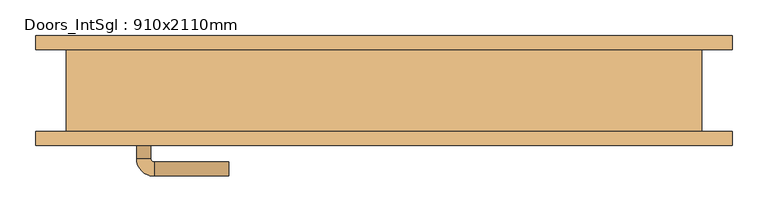
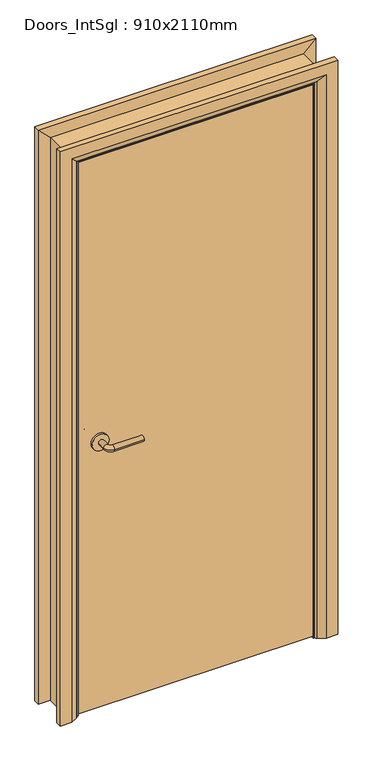
"""IFC4 building model written with IfcOpenShell, lengths in millimetres: door geometry, Doors_IntSgl : 910x2110mm."""

from ifc_helpers import new_model, si_unit, point, frame, frame_2d, origin, place, context, project, spatial, polyline, circle_curve, ellipse_curve, trimmed, segment, composite_curve, outline, extrude, faceted_brep, source, transform, mapped, element, save
from ifc_brep_helpers import plane_surface, cylinder_surface, revolved_surface, advanced_brep


def doors_intsgl_910x2110mm_d0108889(model_context):
    return source(origin(), model_context, "Body", "SolidModel", [
        advanced_brep(
        [(-348.0, -11.5, 1000.0), (-328.0, -11.5, 1000.0), (-348.0, 18.5, 1000.0), (-328.0, 18.5, 1000.0), (-323.0, 23.5, 1000.0), (-323.0, 43.5, 1000.0), (-218.0, 43.5, 1000.0), (-218.0, 23.5, 1000.0)],
        [
            (0, 1, circle_curve(frame((-338.0, -11.5, 1000.0), z_axis=(0.0, -1.0, 0.0), x_axis=(1.0, 0.0, 0.0)), 10.0)),
            (1, 0, circle_curve(frame((-338.0, -11.5, 1000.0), z_axis=(0.0, -1.0, 0.0), x_axis=(1.0, 0.0, 0.0)), 10.0)),
            (0, 2),
            (2, 3, circle_curve(frame((-338.0, 18.5, 1000.0), z_axis=(0.0, -1.0, 0.0), x_axis=(1.0, 0.0, 0.0)), 10.0)),
            (3, 1),
            (3, 2, circle_curve(frame((-338.0, 18.5, 1000.0), z_axis=(0.0, -1.0, 0.0), x_axis=(1.0, 0.0, 0.0)), 10.0)),
            (4, 3, circle_curve(frame((-323.0, 18.5, 1000.0), z_axis=(0.0, 0.0, 1.0), x_axis=(-1.0, 0.0, 0.0)), 5.0)),
            (2, 5, circle_curve(frame((-323.0, 18.5, 1000.0), z_axis=(0.0, 0.0, -1.0), x_axis=(-1.0, 0.0, 0.0)), 25.0)),
            (5, 4, circle_curve(frame((-323.0, 33.5, 1000.0), z_axis=(-1.0, 0.0, 0.0), x_axis=(0.0, -1.0, 0.0)), 10.0)),
            (4, 5, circle_curve(frame((-323.0, 33.5, 1000.0), z_axis=(-1.0, 0.0, 0.0), x_axis=(0.0, -1.0, 0.0)), 10.0)),
            (6, 7, circle_curve(frame((-218.0, 33.5, 1000.0), z_axis=(1.0, 0.0, 0.0), x_axis=(0.0, -1.0, 0.0)), 10.0)),
            (7, 6, circle_curve(frame((-218.0, 33.5, 1000.0), z_axis=(1.0, 0.0, 0.0), x_axis=(0.0, -1.0, 0.0)), 10.0)),
            (5, 6),
            (7, 4),
        ],
        [
            plane_surface(frame((-338.0, -11.5, 1000.0), z_axis=(0.0, -1.0, 0.0), x_axis=(0.0, 0.0, 1.0))),
            cylinder_surface(frame((-338.0, -11.5, 1000.0), z_axis=(0.0, -1.0, 0.0), x_axis=(1.0, 0.0, 0.0)), 10.0),
            revolved_surface(trimmed(ellipse_curve(frame((-338.0, 18.5, 1000.0), z_axis=(0.0, -1.0, 0.0), x_axis=(1.0, 0.0, 0.0)), 10.0, 10.0), [point((-348.0, 18.5, 1000.0))], [point((-328.0, 18.5, 1000.0))], True, "CARTESIAN"), (-323.0, 18.5, 1000.0), (0.0, 0.0, -1.0)),
            revolved_surface(trimmed(ellipse_curve(frame((-338.0, 18.5, 1000.0), z_axis=(0.0, -1.0, 0.0), x_axis=(1.0, 0.0, 0.0)), 10.0, 10.0), [point((-328.0, 18.5, 1000.0))], [point((-348.0, 18.5, 1000.0))], True, "CARTESIAN"), (-323.0, 18.5, 1000.0), (0.0, 0.0, -1.0)),
            plane_surface(frame((-218.0, 33.5, 1000.0), z_axis=(1.0, 0.0, 0.0), x_axis=(0.0, 0.0, 1.0))),
            cylinder_surface(frame((-323.0, 33.5, 1000.0), z_axis=(-1.0, 0.0, 0.0), x_axis=(0.0, -1.0, 0.0)), 10.0),
        ],
        [
            (0, [[1, 2]]),
            (1, [[-1, 3, 4, 5]]),
            (1, [[-2, -5, 6, -3]]),
            (2, [[7, -4, 8, 9]]),
            (3, [[-8, -6, -7, 10]]),
            (4, [[11, 12]]),
            (5, [[-9, 13, -12, 14]]),
            (5, [[-10, -14, -11, -13]]),
        ],
    ),
        extrude(outline(composite_curve([segment(trimmed(circle_curve(frame_2d((1000.0, -340.5)), 30.0), [point((1000.0, -370.5))], [point((1000.0, -310.5))], False, "CARTESIAN"), True, "CONTINUOUS"), segment(trimmed(circle_curve(frame_2d((1000.0, -340.5)), 30.0), [point((1000.0, -310.5))], [point((1000.0, -370.5))], False, "CARTESIAN"), True, "CONTINUOUS")], self_intersect=False)), frame((0.0, -19.5, 0.0), z_axis=(0.0, 1.0, 0.0), x_axis=(0.0, 0.0, 1.0)), (0.0, 0.0, 1.0), 8.0),
        advanced_brep(
        [(-348.0, -65.5, 1000.0), (-328.0, -65.5, 1000.0), (-328.0, -95.5, 1000.0), (-348.0, -95.5, 1000.0), (-323.0, -100.5, 1000.0), (-323.0, -120.5, 1000.0), (-218.0, -120.5, 1000.0), (-218.0, -100.5, 1000.0)],
        [
            (0, 1, circle_curve(frame((-338.0, -65.5, 1000.0), z_axis=(0.0, 1.0, 0.0), x_axis=(1.0, 0.0, 0.0)), 10.0)),
            (1, 0, circle_curve(frame((-338.0, -65.5, 1000.0), z_axis=(0.0, 1.0, 0.0), x_axis=(1.0, 0.0, 0.0)), 10.0)),
            (1, 2),
            (2, 3, circle_curve(frame((-338.0, -95.5, 1000.0), z_axis=(0.0, 1.0, 0.0), x_axis=(1.0, 0.0, 0.0)), 10.0)),
            (3, 0),
            (3, 2, circle_curve(frame((-338.0, -95.5, 1000.0), z_axis=(0.0, 1.0, 0.0), x_axis=(1.0, 0.0, 0.0)), 10.0)),
            (4, 5, circle_curve(frame((-323.0, -110.5, 1000.0), z_axis=(-1.0, 0.0, 0.0), x_axis=(0.0, 1.0, 0.0)), 10.0)),
            (5, 3, circle_curve(frame((-323.0, -95.5, 1000.0), z_axis=(0.0, 0.0, -1.0), x_axis=(-1.0, 0.0, 0.0)), 25.0)),
            (2, 4, circle_curve(frame((-323.0, -95.5, 1000.0), z_axis=(0.0, 0.0, 1.0), x_axis=(-1.0, 0.0, 0.0)), 5.0)),
            (5, 4, circle_curve(frame((-323.0, -110.5, 1000.0), z_axis=(-1.0, 0.0, 0.0), x_axis=(0.0, 1.0, 0.0)), 10.0)),
            (6, 7, circle_curve(frame((-218.0, -110.5, 1000.0), z_axis=(1.0, 0.0, 0.0), x_axis=(0.0, 1.0, 0.0)), 10.0)),
            (7, 6, circle_curve(frame((-218.0, -110.5, 1000.0), z_axis=(1.0, 0.0, 0.0), x_axis=(0.0, 1.0, 0.0)), 10.0)),
            (4, 7),
            (6, 5),
        ],
        [
            plane_surface(frame((-338.0, -65.5, 1000.0), z_axis=(0.0, 1.0, 0.0), x_axis=(0.0, 0.0, 1.0))),
            cylinder_surface(frame((-338.0, -65.5, 1000.0), z_axis=(0.0, 1.0, 0.0), x_axis=(1.0, 0.0, 0.0)), 10.0),
            revolved_surface(trimmed(ellipse_curve(frame((-338.0, -95.5, 1000.0), z_axis=(0.0, -1.0, 0.0), x_axis=(1.0, 0.0, 0.0)), 10.0, 10.0), [point((-348.0, -95.5, 1000.0))], [point((-328.0, -95.5, 1000.0))], True, "CARTESIAN"), (-323.0, -95.5, 1000.0), (0.0, 0.0, -1.0)),
            revolved_surface(trimmed(ellipse_curve(frame((-338.0, -95.5, 1000.0), z_axis=(0.0, -1.0, 0.0), x_axis=(1.0, 0.0, 0.0)), 10.0, 10.0), [point((-328.0, -95.5, 1000.0))], [point((-348.0, -95.5, 1000.0))], True, "CARTESIAN"), (-323.0, -95.5, 1000.0), (0.0, 0.0, -1.0)),
            plane_surface(frame((-218.0, -110.5, 1000.0), z_axis=(1.0, 0.0, 0.0), x_axis=(0.0, 0.0, 1.0))),
            cylinder_surface(frame((-323.0, -110.5, 1000.0), z_axis=(-1.0, 0.0, 0.0), x_axis=(0.0, 1.0, 0.0)), 10.0),
        ],
        [
            (0, [[1, 2]]),
            (1, [[3, 4, 5, -2]]),
            (1, [[-5, 6, -3, -1]]),
            (2, [[7, 8, -4, 9]]),
            (3, [[10, -9, -6, -8]]),
            (4, [[11, 12]]),
            (5, [[13, -11, 14, -7]]),
            (5, [[-14, -12, -13, -10]]),
        ],
    ),
        extrude(outline(composite_curve([segment(trimmed(circle_curve(frame_2d((1000.0, -340.5)), 30.0), [point((1000.0, -370.5))], [point((1000.0, -310.5))], False, "CARTESIAN"), True, "CONTINUOUS"), segment(trimmed(circle_curve(frame_2d((1000.0, -340.5)), 30.0), [point((1000.0, -310.5))], [point((1000.0, -370.5))], False, "CARTESIAN"), True, "CONTINUOUS")], self_intersect=False)), frame((0.0, -65.5, 0.0), z_axis=(0.0, 1.0, 0.0), x_axis=(0.0, 0.0, 1.0)), (0.0, 0.0, 1.0), 8.0),
        extrude(outline(polyline([(413.0, -19.5), (413.0, -57.5), (-413.0, -57.5), (-413.0, -19.5), (413.0, -19.5)])), frame((0.0, 0.0, 8.0), z_axis=(0.0, 0.0, 1.0), x_axis=(1.0, 0.0, 0.0)), (0.0, 0.0, 1.0), 2060.0),
        advanced_brep(
        [(490.0, -77.5, 0.0), (450.0, -77.5, 0.0), (424.0, -63.5, 0.0), (420.0, -57.5, 0.0), (490.0, -57.5, 0.0), (490.0, -57.5, 2145.0), (490.0, -77.5, 2145.0), (420.0, -57.5, 2075.0), (-420.0, -57.5, 2075.0), (-420.0, -57.5, 0.0), (-490.0, -57.5, 0.0), (-490.0, -57.5, 2145.0), (424.0, -63.5, 2079.0), (450.0, -77.5, 2105.0), (-490.0, -77.5, 2145.0), (-490.0, -77.5, 0.0), (-450.0, -77.5, 0.0), (-450.0, -77.5, 2105.0), (-424.0, -63.5, 2079.0), (-424.0, -63.5, 0.0)],
        [
            (0, 1),
            (1, 2),
            (2, 3, circle_curve(frame((428.0, -56.5, 0.0), z_axis=(0.0, 0.0, -1.0), x_axis=(1.0, 0.0, 0.0)), 8.0622577)),
            (3, 4),
            (4, 0),
            (4, 5),
            (5, 6),
            (6, 0),
            (3, 7),
            (7, 8),
            (8, 9),
            (9, 10),
            (10, 11),
            (11, 5),
            (2, 12),
            (12, 7, ellipse_curve(frame((428.0, -56.5, 2083.0), z_axis=(0.7071067811865475, 0.0, -0.7071067811865475), x_axis=(-0.7071067811865474, 0.0, -0.7071067811865476)), 11.4017543, 8.0622577)),
            (1, 13),
            (13, 12),
            (6, 14),
            (14, 15),
            (15, 16),
            (16, 17),
            (17, 13),
            (11, 14),
            (12, 18),
            (18, 8, ellipse_curve(frame((-428.0, -56.5, 2083.0), z_axis=(0.7071067811865475, 0.0, 0.7071067811865475), x_axis=(0.7071067811865476, 0.0, -0.7071067811865474)), 11.4017543, 8.0622577)),
            (17, 18),
            (15, 10),
            (9, 19, circle_curve(frame((-428.0, -56.5, 0.0), z_axis=(0.0, 0.0, -1.0), x_axis=(-1.0, 0.0, 0.0)), 8.0622577)),
            (19, 16),
            (18, 19),
        ],
        [
            plane_surface(frame((420.0, -57.5, 0.0), z_axis=(0.0, 0.0, -1.0), x_axis=(0.0, 1.0, 0.0))),
            plane_surface(frame((490.0, -77.5, 0.0), z_axis=(1.0, 0.0, 0.0), x_axis=(0.0, 0.0, 1.0))),
            plane_surface(frame((490.0, -57.5, 0.0), z_axis=(0.0, 1.0, 0.0), x_axis=(0.0, 0.0, 1.0))),
            cylinder_surface(frame((428.0, -56.5, 0.0), z_axis=(0.0, 0.0, -1.0), x_axis=(1.0, 0.0, 0.0)), 8.0622577),
            plane_surface(frame((424.0, -63.5, 0.0), z_axis=(-0.4740998230350126, -0.880471099922178, 0.0), x_axis=(0.0, 0.0, 1.0))),
            plane_surface(frame((450.0, -77.5, 0.0), z_axis=(0.0, -1.0, 0.0), x_axis=(0.0, 0.0, 1.0))),
            plane_surface(frame((490.0, -77.5, 2145.0), z_axis=(0.0, 0.0, 1.0), x_axis=(-1.0, 0.0, 0.0))),
            cylinder_surface(frame((420.0, -56.5, 2083.0), z_axis=(1.0, 0.0, 0.0), x_axis=(0.0, 0.0, 1.0)), 8.0622577),
            plane_surface(frame((424.0, -63.5, 2079.0), z_axis=(0.0, -0.8804710999221764, -0.4740998230350154), x_axis=(-1.0, 0.0, 0.0))),
            plane_surface(frame((-420.0, -57.5, 0.0), z_axis=(0.0, 0.0, -1.0), x_axis=(0.0, 1.0, 0.0))),
            plane_surface(frame((-490.0, -77.5, 2145.0), z_axis=(-1.0, 0.0, 0.0), x_axis=(0.0, 0.0, -1.0))),
            cylinder_surface(frame((-428.0, -56.5, 2075.0), z_axis=(0.0, 0.0, 1.0), x_axis=(-1.0, 0.0, 0.0)), 8.0622577),
            plane_surface(frame((-424.0, -63.5, 2079.0), z_axis=(0.47409982303501824, -0.8804710999221749, 0.0), x_axis=(0.0, 0.0, -1.0))),
        ],
        [
            (0, [[1, 2, 3, 4, 5]]),
            (1, [[6, 7, 8, -5]]),
            (2, [[9, 10, 11, 12, 13, 14, -6, -4]]),
            (3, [[15, 16, -9, -3]]),
            (4, [[17, 18, -15, -2]]),
            (5, [[-8, 19, 20, 21, 22, 23, -17, -1]]),
            (6, [[-14, 24, -19, -7]]),
            (7, [[25, 26, -10, -16]]),
            (8, [[-23, 27, -25, -18]]),
            (9, [[28, -12, 29, 30, -21]]),
            (10, [[-13, -28, -20, -24]]),
            (11, [[31, -29, -11, -26]]),
            (12, [[-22, -30, -31, -27]]),
        ],
    ),
        extrude(outline(polyline([(0.0, -396.0), (2051.0, -396.0), (2051.0, 396.0), (0.0, 396.0), (0.0, 415.0), (2070.0, 415.0), (2070.0, -415.0), (0.0, -415.0), (0.0, -396.0)])), frame((0.0, -17.5, 0.0), z_axis=(0.0, 1.0, 0.0), x_axis=(0.0, 0.0, 1.0)), (0.0, 0.0, 1.0), 32.0),
        advanced_brep(
        [(-490.0, 77.5, 0.0), (-450.0, 77.5, 0.0), (-424.0, 63.5, 0.0), (-420.0, 57.5, 0.0), (-490.0, 57.5, 0.0), (-490.0, 57.5, 2145.0), (-490.0, 77.5, 2145.0), (-420.0, 57.5, 2075.0), (-424.0, 63.5, 2079.0), (-450.0, 77.5, 2105.0), (490.0, 57.5, 2145.0), (490.0, 77.5, 2145.0), (420.0, 57.5, 2075.0), (424.0, 63.5, 2079.0), (450.0, 77.5, 2105.0), (490.0, 77.5, 0.0), (490.0, 57.5, 0.0), (420.0, 57.5, 0.0), (424.0, 63.5, 0.0), (450.0, 77.5, 0.0)],
        [
            (0, 1),
            (1, 2),
            (2, 3, circle_curve(frame((-428.0, 56.5, 0.0), z_axis=(0.0, 0.0, -1.0), x_axis=(-1.0, 0.0, 0.0)), 8.0622577)),
            (3, 4),
            (4, 0),
            (4, 5),
            (5, 6),
            (6, 0),
            (3, 7),
            (7, 5),
            (2, 8),
            (8, 7, ellipse_curve(frame((-428.0, 56.5, 2083.0), z_axis=(-0.7071067811865475, 0.0, -0.7071067811865475), x_axis=(0.7071067811865474, 0.0, -0.7071067811865476)), 11.4017543, 8.0622577)),
            (1, 9),
            (9, 8),
            (6, 9),
            (5, 10),
            (10, 11),
            (11, 6),
            (7, 12),
            (12, 10),
            (8, 13),
            (13, 12, ellipse_curve(frame((428.0, 56.5, 2083.0), z_axis=(-0.7071067811865475, 0.0, 0.7071067811865475), x_axis=(-0.7071067811865476, 0.0, -0.7071067811865474)), 11.4017543, 8.0622577)),
            (9, 14),
            (14, 13),
            (11, 14),
            (15, 16),
            (16, 17),
            (17, 18, circle_curve(frame((428.0, 56.5, 0.0), z_axis=(0.0, 0.0, -1.0), x_axis=(1.0, 0.0, 0.0)), 8.0622577)),
            (18, 19),
            (19, 15),
            (10, 16),
            (15, 11),
            (12, 17),
            (13, 18),
            (14, 19),
        ],
        [
            plane_surface(frame((-420.0, 130.3010989, 0.0), z_axis=(0.0, 0.0, -1.0), x_axis=(1.0, 0.0, 0.0))),
            plane_surface(frame((-490.0, 77.5, 0.0), z_axis=(-1.0, 0.0, 0.0), x_axis=(0.0, 0.0, 1.0))),
            plane_surface(frame((-490.0, 57.5, 0.0), z_axis=(0.0, -1.0, 0.0), x_axis=(0.0, 0.0, 1.0))),
            cylinder_surface(frame((-428.0, 56.5, 0.0), z_axis=(0.0, 0.0, -1.0), x_axis=(-1.0, 0.0, 0.0)), 8.0622577),
            plane_surface(frame((-424.0, 63.5, 0.0), z_axis=(0.4740998230350183, 0.8804710999221749, 0.0), x_axis=(0.0, 0.0, 1.0))),
            plane_surface(frame((-450.0, 77.5, 0.0), z_axis=(0.0, 1.0, 0.0), x_axis=(0.0, 0.0, 1.0))),
            plane_surface(frame((-490.0, 77.5, 2145.0), z_axis=(0.0, 0.0, 1.0), x_axis=(1.0, 0.0, 0.0))),
            plane_surface(frame((-490.0, 57.5, 2145.0), z_axis=(0.0, -1.0, 0.0), x_axis=(1.0, 0.0, 0.0))),
            cylinder_surface(frame((-420.0, 56.5, 2083.0), z_axis=(-1.0, 0.0, 0.0), x_axis=(0.0, 0.0, 1.0)), 8.0622577),
            plane_surface(frame((-424.0, 63.5, 2079.0), z_axis=(0.0, 0.8804710999221749, -0.4740998230350183), x_axis=(1.0, 0.0, 0.0))),
            plane_surface(frame((-450.0, 77.5, 2105.0), z_axis=(0.0, 1.0, 0.0), x_axis=(1.0, 0.0, 0.0))),
            plane_surface(frame((420.0, 130.3010989, 0.0), z_axis=(0.0, 0.0, -1.0), x_axis=(-1.0, 0.0, 0.0))),
            plane_surface(frame((490.0, 77.5, 2145.0), z_axis=(1.0, 0.0, 0.0), x_axis=(0.0, 0.0, -1.0))),
            plane_surface(frame((490.0, 57.5, 2145.0), z_axis=(0.0, -1.0, 0.0), x_axis=(0.0, 0.0, -1.0))),
            cylinder_surface(frame((428.0, 56.5, 2075.0), z_axis=(0.0, 0.0, 1.0), x_axis=(1.0, 0.0, 0.0)), 8.0622577),
            plane_surface(frame((424.0, 63.5, 2079.0), z_axis=(-0.4740998230350183, 0.8804710999221749, 0.0), x_axis=(0.0, 0.0, -1.0))),
            plane_surface(frame((450.0, 77.5, 2105.0), z_axis=(0.0, 1.0, 0.0), x_axis=(0.0, 0.0, -1.0))),
        ],
        [
            (0, [[1, 2, 3, 4, 5]]),
            (1, [[6, 7, 8, -5]]),
            (2, [[9, 10, -6, -4]]),
            (3, [[11, 12, -9, -3]]),
            (4, [[13, 14, -11, -2]]),
            (5, [[-8, 15, -13, -1]]),
            (6, [[16, 17, 18, -7]]),
            (7, [[19, 20, -16, -10]]),
            (8, [[21, 22, -19, -12]]),
            (9, [[23, 24, -21, -14]]),
            (10, [[-18, 25, -23, -15]]),
            (11, [[26, 27, 28, 29, 30]]),
            (12, [[31, -26, 32, -17]]),
            (13, [[33, -27, -31, -20]]),
            (14, [[34, -28, -33, -22]]),
            (15, [[35, -29, -34, -24]]),
            (16, [[-32, -30, -35, -25]]),
        ],
    ),
        faceted_brep([(-415.0, -57.5, 0.0), (-447.0, -57.5, 0.0), (-447.0, 57.5, 0.0), (-415.0, 57.5, 0.0), (-415.0, 57.5, 2070.0), (-415.0, -57.5, 2070.0), (-447.0, 57.5, 2102.0), (-447.0, -57.5, 2102.0), (415.0, 57.5, 2070.0), (415.0, -57.5, 2070.0), (447.0, 57.5, 2102.0), (447.0, -57.5, 2102.0), (415.0, -57.5, 0.0), (415.0, 57.5, 0.0), (447.0, 57.5, 0.0), (447.0, -57.5, 0.0)], [[[0, 1, 2, 3]], [[3, 4, 5, 0]], [[2, 6, 4, 3]], [[1, 7, 6, 2]], [[0, 5, 7, 1]], [[4, 8, 9, 5]], [[6, 10, 8, 4]], [[7, 11, 10, 6]], [[5, 9, 11, 7]], [[12, 13, 14, 15]], [[8, 13, 12, 9]], [[10, 14, 13, 8]], [[11, 15, 14, 10]], [[9, 12, 15, 11]]]),
    ])


if __name__ == "__main__":
    model = new_model("IFC4")
    model_context = context("Model", 3, world=origin())
    ifc_project = project(units=[si_unit("LENGTHUNIT", "METRE", prefix="MILLI")], contexts=[model_context])
    site = spatial("IfcSite", under=ifc_project)
    building = spatial("IfcBuilding", under=site)
    placement = place(None, origin())
    doors_intsgl_910x2110mm_shape = doors_intsgl_910x2110mm_d0108889(model_context)
    element("IfcDoor", 1, ObjectType="Doors_IntSgl : 910x2110mm", at=placement, inside=building, context=model_context, shape_type="MappedRepresentation", body=[
        mapped(doors_intsgl_910x2110mm_shape, transform((0.0, 0.0, 0.0), x_axis=(1.0, 0.0, 0.0), y_axis=(0.0, 1.0, 0.0), z_axis=(0.0, 0.0, 1.0))),
    ])
    save(model, "model.ifc")

# Revit data of these elements
# Type "Doors_IntSgl : 910x2110mm"
#   Construction Type Id = "MDOOR"
#   Type Mark = "41"
#   Type Comments = "Internal Single"
#   Operation = "SingleSwingRight"
#   Manufacturer = "Revit"
#   Keynote = "L20"
#   Description = "Internal Single Door"
#   Analytic Construction = "Metal"
#   UnderCut = 8 mm
#   Tolerance = 2 mm
#   Thickness = 38 mm
#   Thermal Resistance (R) = 0.270117 (m²·K)/W
#   Structural Tolerance = 8 mm
#   StopDepth = 32 mm
#   Stop Thickness = 19 mm
#   Rough Width = 910 mm
#   Rough Height = 2110 mm
#   Height to Top Lock Rail = 1000 mm
#   Heat Transfer Coefficient (U) = 3.7021 W/(m²·K)
#   Handle Z Distance = 1000 mm
#   Handle X Distance = 75 mm
#   Frame Thickness = 32 mm
#   Door Panel Width = 826 mm
#   Door Panel Thickness = 38 mm
#   Door Panel Offset = 0 mm
#   Height = 2110 mm
#   Width = 910 mm
#   Door Panel Height = 2060 mm
#   Architrave Setback = 5 mm
#   Define Thermal Properties by = 1
#   Vis - Ironmongery = yes
#   Material Ironmongery = Door - Handle
#   Material Frame = Door - Frame/Mullion (1)
#   Material Door = Door - Panel
#   Material Architrave = Door - Architrave
#   Visual Light Transmittance = 0
#   Solar Heat Gain Coefficient = 0
#   Function = (empty or 0)
#   Wall Closure = (empty or 0)
# Element 1 (IfcDoor, "Doors_IntSgl : 910x2110mm")
#   Materials on its faces: "Door - Architrave", "Door - Handle", "Door - Frame/Mullion (1)", "Door - Panel"
# Materials
#   "Door - Handle": class "Miscellaneous", colour RGB 0 0 0, transparency 0, Keynote = "P21", Cost = 0
#   "Door - Frame/Mullion (1)": class "Wood", colour RGB 212 179 113, transparency 0, Keynote = "L20", Cost = 0
#   "Door - Panel": class "Wood", colour RGB 210 159 95, transparency 0, Keynote = "L20", Cost = 0
#   "Door - Architrave": class "Wood", colour RGB 154 90 5, transparency 0, Keynote = "P20", Cost = 0
